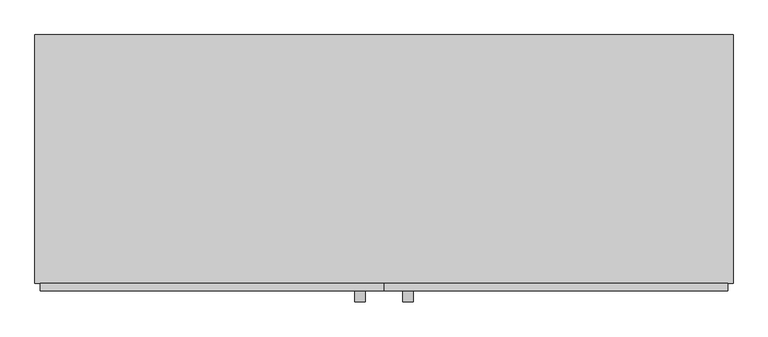
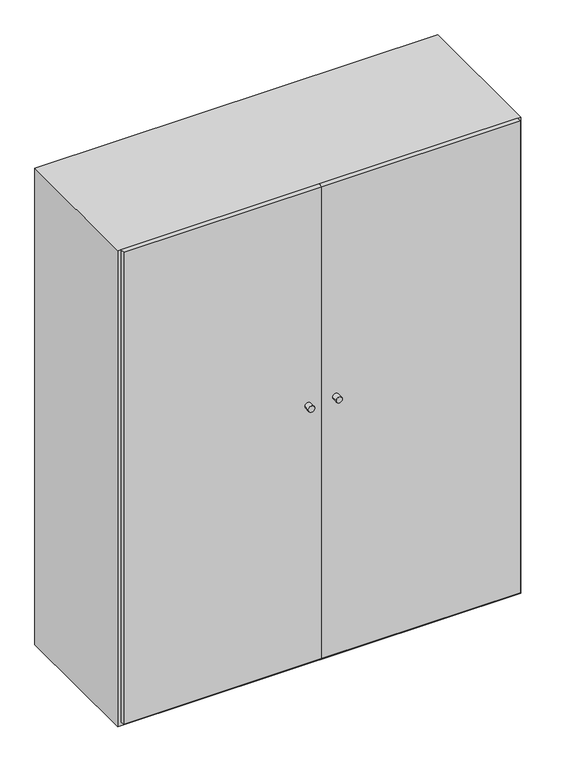
"""IFC4 building model written with IfcOpenShell, lengths in millimetres: furniture geometry, Armario dormitorio : ARMARIO DORM_PABLO."""

from ifc_helpers import new_model, si_unit, point, frame, frame_2d, origin, origin_with_axes, place, context, project, spatial, polyline, circle_curve, trimmed, segment, composite_curve, outline, extrude, source, transform, mapped, element, save


def furniture_64353a5b(model_context):
    return source(origin(), model_context, "Body", "SweptSolid", [
        extrude(outline(composite_curve([segment(trimmed(circle_curve(frame_2d((1100.0, -55.0)), 12.5), [point((1100.0, -67.5))], [point((1100.0, -42.5))], False, "CARTESIAN"), True, "CONTINUOUS"), segment(trimmed(circle_curve(frame_2d((1100.0, -55.0)), 12.5), [point((1100.0, -42.5))], [point((1100.0, -67.5))], False, "CARTESIAN"), True, "CONTINUOUS")], self_intersect=False)), frame((0.0, -613.0, 0.0), z_axis=(0.0, 1.0, 0.0), x_axis=(0.0, 0.0, 1.0)), (0.0, 0.0, 1.0), 25.0),
        extrude(outline(composite_curve([segment(trimmed(circle_curve(frame_2d((1100.0, 55.0)), 12.5), [point((1100.0, 42.5))], [point((1100.0, 67.5))], False, "CARTESIAN"), True, "CONTINUOUS"), segment(trimmed(circle_curve(frame_2d((1100.0, 55.0)), 12.5), [point((1100.0, 67.5))], [point((1100.0, 42.5))], False, "CARTESIAN"), True, "CONTINUOUS")], self_intersect=False)), frame((0.0, -613.0, 0.0), z_axis=(0.0, 1.0, 0.0), x_axis=(0.0, 0.0, 1.0)), (0.0, 0.0, 1.0), 25.0),
        extrude(outline(polyline([(0.0, -570.0), (787.5, -570.0), (787.5, -588.0), (0.0, -588.0), (0.0, -570.0)])), frame((0.0, 0.0, 18.0), z_axis=(0.0, 0.0, 1.0), x_axis=(1.0, 0.0, 0.0)), (0.0, 0.0, 1.0), 1982.0),
        extrude(outline(polyline([(0.0, -570.0), (0.0, -588.0), (-787.5, -588.0), (-787.5, -570.0), (0.0, -570.0)])), frame((0.0, 0.0, 18.0), z_axis=(0.0, 0.0, 1.0), x_axis=(1.0, 0.0, 0.0)), (0.0, 0.0, 1.0), 1982.0),
        extrude(outline(polyline([(800.0, 0.0), (800.0, -570.0), (-800.0, -570.0), (-800.0, 0.0), (800.0, 0.0)])), origin_with_axes(), (0.0, 0.0, 1.0), 2000.0),
    ])


if __name__ == "__main__":
    model = new_model("IFC4")
    model_context = context("Model", 3, world=origin())
    ifc_project = project(units=[si_unit("LENGTHUNIT", "METRE", prefix="MILLI")], contexts=[model_context])
    site = spatial("IfcSite", under=ifc_project)
    building = spatial("IfcBuilding", under=site)
    placement = place(None, origin())
    furniture_shape = furniture_64353a5b(model_context)
    element("IfcFurniture", 1, ObjectType="Armario dormitorio : ARMARIO DORM_PABLO", at=placement, inside=building, context=model_context, shape_type="MappedRepresentation", body=[
        mapped(furniture_shape, transform((0.0, 0.0, 0.0), x_axis=(1.0, 0.0, 0.0), y_axis=(0.0, 1.0, 0.0), z_axis=(0.0, 0.0, 1.0))),
    ])
    save(model, "model.ifc")

# Revit data of these elements
# Type "Armario dormitorio : ARMARIO DORM_PABLO"
#   Anchura = 1.60 m
#   Altura = 2.00 m
#   Profundidad = 0.57 m
#   Material de armario = none
#   Default Elevation = 0
# Element 1 (IfcFurniture, "Armario dormitorio : ARMARIO DORM_PABLO")
#   Materials on its faces: "Madera - Listel"
# Materials
#   "Madera - Listel": class "Madera", colour RGB 210 180 110, transparency 0, Cost = 0
